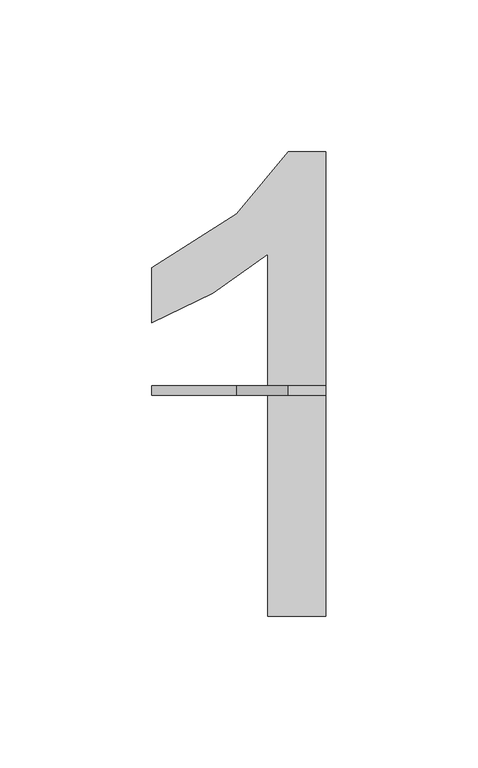
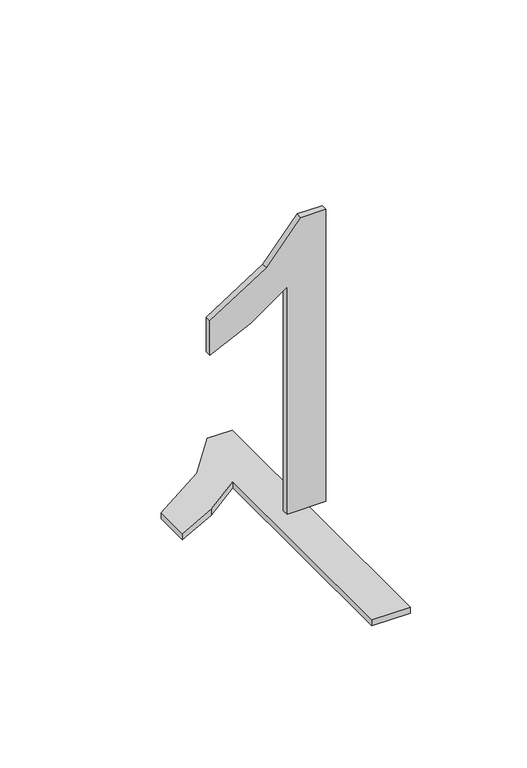
"""IFC4 building model written with IfcOpenShell, lengths in millimetres: proxy geometry, Grid Number1_FedEx : Grid Number1_FedEx."""

from ifc_helpers import new_model, si_unit, frame, origin, origin_with_axes, place, context, project, spatial, polyline, outline, extrude, source, transform, mapped, element, save


def entourage_6be843fa(model_context):
    return source(origin(), model_context, "Body", "SweptSolid", [
        extrude(outline(polyline([(-85.3488258, 146.5840649), (-104.4857529, 146.5840649), (-104.4857529, 265.8908447), (-122.6135061, 252.9771566), (-142.7596071, 243.315251), (-142.7596071, 261.4056274), (-114.7083106, 279.3091198), (-97.6831734, 299.6794816), (-85.3488258, 299.6794816), (-85.3488258, 146.5840649)])), origin_with_axes(), (0.0, 0.0, 1.0), 3.175),
        extrude(outline(polyline([(14.4798932, -85.3488258), (167.5753099, -85.3488258), (167.5753099, -97.6831734), (147.2049481, -114.7083106), (129.3014557, -142.7596071), (111.2110794, -142.7596071), (120.8729849, -122.6135061), (133.786673, -104.4857529), (14.4798932, -104.4857529), (14.4798932, -85.3488258)])), frame((0.0, 219.3456765, 0.0), z_axis=(0.0, 1.0, 0.0), x_axis=(0.0, 0.0, 1.0)), (0.0, 0.0, 1.0), 3.175),
    ])


if __name__ == "__main__":
    model = new_model("IFC4")
    model_context = context("Model", 3, world=origin())
    ifc_project = project(units=[si_unit("LENGTHUNIT", "METRE", prefix="MILLI")], contexts=[model_context])
    site = spatial("IfcSite", under=ifc_project)
    building = spatial("IfcBuilding", under=site)
    placement = place(None, origin())
    entourage_shape = entourage_6be843fa(model_context)
    element("IfcBuildingElementProxy", 1, Name="Grid Number1_FedEx : Grid Number1_FedEx", ObjectType="Grid Number1_FedEx : Grid Number1_FedEx", at=placement, inside=building, context=model_context, shape_type="MappedRepresentation", body=[
        mapped(entourage_shape, transform((0.0, 0.0, 0.0), x_axis=(1.0, 0.0, 0.0), y_axis=(0.0, 1.0, 0.0), z_axis=(0.0, 0.0, 1.0))),
    ])
    save(model, "model.ifc")

# Revit data of these elements
# Type "Grid Number1_FedEx : Grid Number1_FedEx"
#   Grid [instance default] = "S.8"
#   Label Width [instance default] = 1' - 0"
#   Half Box Width2 [instance default] = 0' - 6.13846"
#   Half Box Width [instance default] = 0' - 6"
#   Robust [instance default] = yes
#   Height = 0
#   Assembly Code = ""
# Element 1 (IfcBuildingElementProxy, "Grid Number1_FedEx : Grid Number1_FedEx")
#   Grid = "1"
#   Robust = no
#   Materials on its faces: "Letter"
# Materials
#   "Letter": class "Unassigned", colour RGB 178 187 30, transparency 0, Comments = "Rendering appearance not upgraded "
